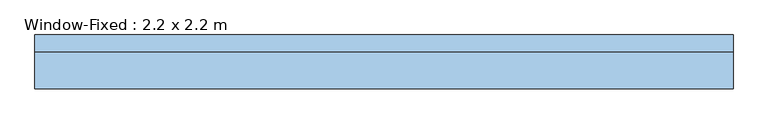
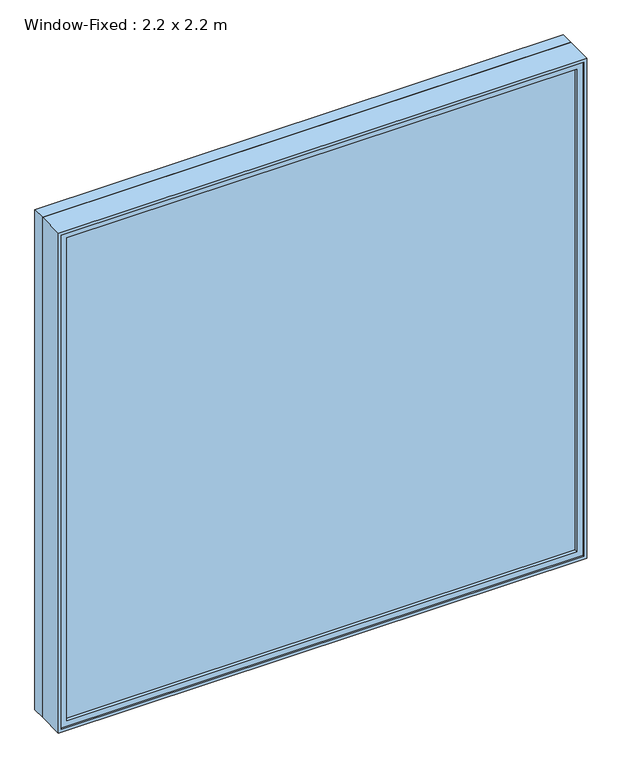
"""IFC4 building model written with IfcOpenShell, lengths in millimetres: window geometry, Window-Fixed : 2.2 x 2.2 m."""

from ifc_helpers import new_model, si_unit, frame, origin, place, context, project, spatial, polyline, outline, extrude, faceted_brep, source, transform, mapped, element, save


def window_fixed_2_2_x_2_2_m_19ca81df(model_context):
    return source(origin(), model_context, "Body", "SolidModel", [
        faceted_brep([(1100.0, 20.25, 3114.4), (-1100.0, 20.25, 3114.4), (-1100.0, -94.05, 3114.4), (1100.0, -94.05, 3114.4), (-1100.0, 20.25, 914.4), (-1100.0, -94.05, 914.4), (1100.0, 20.25, 914.4), (1100.0, -94.05, 914.4), (1068.25, 20.25, 3082.65), (-1068.25, 20.25, 3082.65), (-1068.25, 20.25, 946.15), (1068.25, 20.25, 946.15), (-1087.3, -94.05, 3101.7), (1087.3, -94.05, 3101.7), (1087.3, -94.05, 927.1), (-1087.3, -94.05, 927.1), (1068.25, -43.25, 3082.65), (-1068.25, -43.25, 3082.65), (-1087.3, -43.25, 3101.7), (1087.3, -43.25, 3101.7), (-1068.25, -43.25, 946.15), (-1087.3, -43.25, 927.1), (1068.25, -43.25, 946.15), (1087.3, -43.25, 927.1)], [[[0, 1, 2, 3]], [[1, 4, 5, 2]], [[4, 6, 7, 5]], [[1, 0, 6, 4], [8, 9, 10, 11]], [[6, 0, 3, 7]], [[3, 2, 5, 7], [12, 13, 14, 15]], [[16, 17, 9, 8]], [[13, 12, 18, 19]], [[17, 20, 10, 9]], [[12, 15, 21, 18]], [[20, 22, 11, 10]], [[15, 14, 23, 21]], [[22, 16, 8, 11]], [[19, 18, 21, 23], [17, 16, 22, 20]], [[14, 13, 19, 23]]]),
        extrude(outline(polyline([(3114.4, -1100.0), (914.4, -1100.0), (914.4, 1100.0), (3114.4, 1100.0), (3114.4, -1100.0)]), holes=[polyline([(3101.7, 1087.3), (927.1, 1087.3), (927.1, -1087.3), (3101.7, -1087.3), (3101.7, 1087.3)])]), frame((0.0, 20.25, 0.0), z_axis=(0.0, 1.0, 0.0), x_axis=(0.0, 0.0, 1.0)), (0.0, 0.0, 1.0), 54.75),
        extrude(outline(polyline([(927.1, -1087.3), (927.1, 1087.3), (3101.7, 1087.3), (3101.7, -1087.3), (927.1, -1087.3)]), holes=[polyline([(952.5, 1061.9), (952.5, -1061.9), (3076.3, -1061.9), (3076.3, 1061.9), (952.5, 1061.9)])]), frame((0.0, -87.7, 0.0), z_axis=(0.0, 1.0, 0.0), x_axis=(0.0, 0.0, 1.0)), (0.0, 0.0, 1.0), 44.45),
        extrude(outline(polyline([(1061.9, -75.0), (-1061.9, -75.0), (-1061.9, -68.65), (1061.9, -68.65), (1061.9, -75.0)])), frame((0.0, 0.0, 952.5), z_axis=(0.0, 0.0, 1.0), x_axis=(1.0, 0.0, 0.0)), (0.0, 0.0, 1.0), 2123.8),
        extrude(outline(polyline([(-1061.9, -55.95), (1061.9, -55.95), (1061.9, -62.3), (-1061.9, -62.3), (-1061.9, -55.95)])), frame((0.0, 0.0, 952.5), z_axis=(0.0, 0.0, 1.0), x_axis=(1.0, 0.0, 0.0)), (0.0, 0.0, 1.0), 2123.8),
    ])


if __name__ == "__main__":
    model = new_model("IFC4")
    model_context = context("Model", 3, world=origin())
    ifc_project = project(units=[si_unit("LENGTHUNIT", "METRE", prefix="MILLI")], contexts=[model_context])
    site = spatial("IfcSite", under=ifc_project)
    building = spatial("IfcBuilding", under=site)
    placement = place(None, origin())
    window_fixed_2_2_x_2_2_m_shape = window_fixed_2_2_x_2_2_m_19ca81df(model_context)
    element("IfcWindow", 1, ObjectType="Window-Fixed : 2.2 x 2.2 m", at=placement, inside=building, context=model_context, shape_type="MappedRepresentation", body=[
        mapped(window_fixed_2_2_x_2_2_m_shape, transform((0.0, 0.0, 0.0), x_axis=(1.0, 0.0, 0.0), y_axis=(0.0, 1.0, 0.0), z_axis=(0.0, 0.0, 1.0))),
    ])
    save(model, "model.ifc")

# Revit data of these elements
# Type "Window-Fixed : 2.2 x 2.2 m"
#   Type Mark = "44"
#   Fire Rating = "0.5h"
#   Analytic Construction = "Double glazing - domestic"
#   Window Inset [instance default] = 0 m
#   Wall Thickness [instance default] = 0.1524 m
#   Visual Light Transmittance = 0.81
#   Thermal Resistance (R) = 0.319569 (m²·K)/W
#   Solar Heat Gain Coefficient = 0.76
#   Rough Width = 2.2127 m
#   Rough Height = 2.2127 m
#   Interior Wall Closure [instance default] = 0.05715 m
#   Height = 2.2 m
#   Heat Transfer Coefficient (U) = 3.12929 W/(m²·K)
#   Frame Extension [instance default] = 0.00635 m
#   Exterior Wall Closure [instance default] = 0.03175 m
#   Extension Jamb [instance default] = 0.05715 m
#   Default Sill Height = 0.9144 m
#   Width = 2.2 m
#   Muntin Visibility = yes
#   Interior Trim Visibility [instance default] = yes
#   Exterior Trim Visibility [instance default] = yes
#   Extension Jamb Visibility [instance default] = yes
#   Muntin Pattern = Muntin Pattern_2x2 : Muntin Pattern_2x2
#   Interior Trim Material = Wood - Stained
#   Interior Trim = Trim-Window-Interior-Flat : Picture Frame
#   Interior Frame Material = Wood - Stained
#   Glass Panel Material = Glass
#   Exterior Trim Material = Clad - White
#   Exterior Trim = Trim-Window-Exterior-Flat : with Sill
#   Exterior Frame Material = Clad - White
#   Wall Closure = (empty or 0)
# Element 1 (IfcWindow, "Window-Fixed : 2.2 x 2.2 m")
#   Wall Thickness = 0.15 m
#   Interior Wall Closure = 0.0572 m
#   Exterior Wall Closure = 0.0318 m
#   Extension Jamb = 0.05475 m
#   Materials on its faces: "Wood - Stained", "Glass", "Clad - White"
# Materials
#   "Wood - Stained": class "Wood", colour RGB 227 170 128, transparency 0, Cost = 0
#   "Glass": class "Glass", colour RGB 0 0 255, transparency 0.75, Description = "Soda Lime Glass", Cost = 0
#   "Clad - White": class "Wood", colour RGB 242 242 238, transparency 0, Cost = 0
